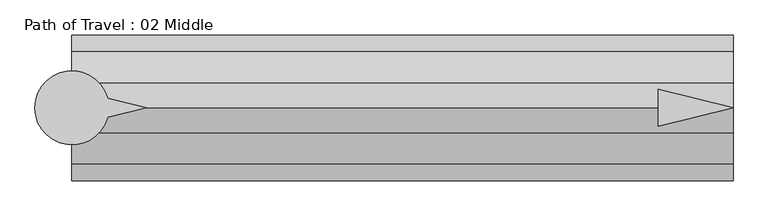
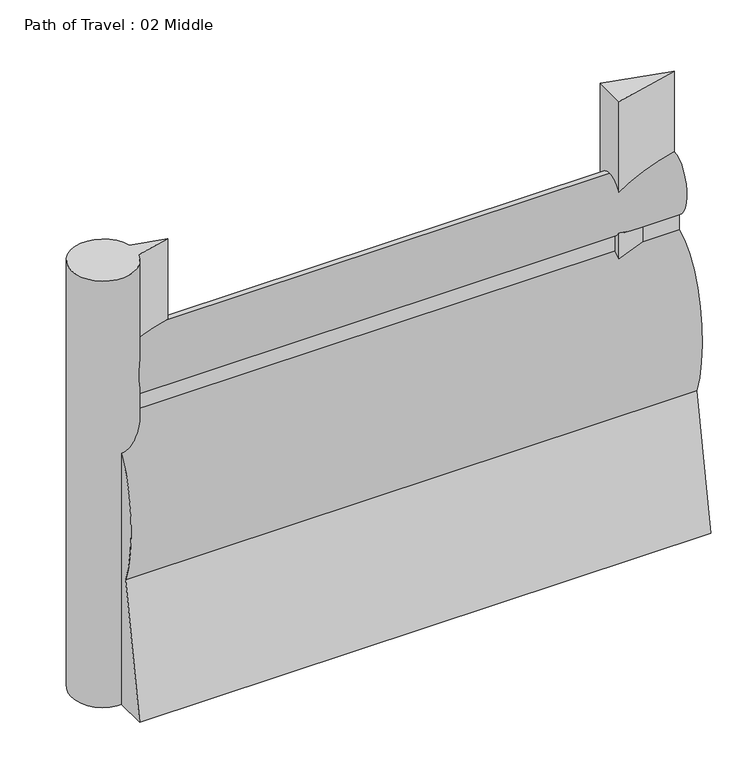
"""IFC4 building model written with IfcOpenShell, lengths in millimetres: proxy geometry, Path of Travel : 02 Middle."""

from ifc_helpers import new_model, si_unit, point, frame, frame_2d, origin, origin_with_axes, place, context, project, spatial, polyline, circle_curve, ellipse_curve, trimmed, segment, composite_curve, outline, extrude, source, transform, mapped, element, save
from ifc_brep_helpers import plane_surface, extruded_surface, advanced_brep


def path_of_travel_02_middle_6eefbcf4(model_context):
    return source(origin(), model_context, "Body", "SolidModel", [
        advanced_brep(
        [(227.5554837, 0.0, 1727.2), (227.5554837, 42.9018657, 1436.6534209), (227.5554837, 42.9018657, 1363.4763406), (227.5554837, 184.1186263, 643.4144547), (227.5554837, 297.5699544, 0.0), (227.5554837, 145.6574193, 0.0), (227.5554837, 0.0, 584.2), (227.5554837, -145.6574193, 0.0), (227.5554837, -297.5699544, 0.0), (227.5554837, -184.1186263, 643.4144547), (227.5554837, -42.9018657, 1363.4763406), (227.5554837, -42.9018657, 1436.6534209), (2925.8453525, 0.0, 1727.2), (2925.8453525, -42.9018657, 1436.6534209), (2925.8453525, -42.9018657, 1363.4763406), (2925.8453525, -184.1186263, 643.4144547), (2925.8453525, -297.5699544, 0.0), (2925.8453525, -145.6574193, 0.0), (2925.8453525, 0.0, 584.2), (2925.8453525, 145.6574193, 0.0), (2925.8453525, 297.5699544, 0.0), (2925.8453525, 184.1186263, 643.4144547), (2925.8453525, 42.9018657, 1363.4763406), (2925.8453525, 42.9018657, 1436.6534209)],
        [
            (0, 1, ellipse_curve(frame((227.5554837, 0.0, 1574.8), z_axis=(-1.0, 0.0, 0.0), x_axis=(0.0, 0.0, 1.0)), 152.4, 101.6)),
            (1, 2),
            (2, 3, ellipse_curve(frame((227.5554837, 0.0, 914.4), z_axis=(-1.0, 0.0, 0.0), x_axis=(0.0, 0.0, -1.0)), 457.2, 228.6)),
            (3, 4),
            (4, 5),
            (5, 6),
            (6, 7),
            (7, 8),
            (8, 9),
            (9, 10, ellipse_curve(frame((227.5554837, 0.0, 914.4), z_axis=(-1.0, 0.0, 0.0), x_axis=(0.0, 0.0, -1.0)), 457.2, 228.6)),
            (10, 11),
            (11, 0, ellipse_curve(frame((227.5554837, 0.0, 1574.8), z_axis=(-1.0, 0.0, 0.0), x_axis=(0.0, 0.0, 1.0)), 152.4, 101.6)),
            (12, 13, ellipse_curve(frame((2925.8453525, 0.0, 1574.8), z_axis=(1.0, 0.0, 0.0), x_axis=(0.0, 0.0, 1.0)), 152.4, 101.6)),
            (13, 14),
            (14, 15, ellipse_curve(frame((2925.8453525, 0.0, 914.4), z_axis=(1.0, 0.0, 0.0), x_axis=(0.0, 0.0, -1.0)), 457.2, 228.6)),
            (15, 16),
            (16, 17),
            (17, 18),
            (18, 19),
            (19, 20),
            (20, 21),
            (21, 22, ellipse_curve(frame((2925.8453525, 0.0, 914.4), z_axis=(1.0, 0.0, 0.0), x_axis=(0.0, 0.0, -1.0)), 457.2, 228.6)),
            (22, 23),
            (23, 12, ellipse_curve(frame((2925.8453525, 0.0, 1574.8), z_axis=(1.0, 0.0, 0.0), x_axis=(0.0, 0.0, 1.0)), 152.4, 101.6)),
            (0, 12),
            (23, 1),
            (22, 2),
            (21, 3),
            (20, 4),
            (19, 5),
            (18, 6),
            (17, 7),
            (16, 8),
            (15, 9),
            (14, 10),
            (13, 11),
        ],
        [
            plane_surface(frame((227.5554837, 0.0, 0.0), z_axis=(-1.0, 0.0, 0.0), x_axis=(0.0, 0.0, 1.0))),
            plane_surface(frame((2925.8453525, 0.0, 0.0), z_axis=(1.0, 0.0, 0.0), x_axis=(0.0, 0.0, 1.0))),
            extruded_surface(trimmed(ellipse_curve(frame((2925.8453525, 0.0, 1574.8), z_axis=(-1.0, 0.0, 0.0), x_axis=(0.0, 0.0, 1.0)), 152.4, 101.6), [point((2925.8453525, 0.0, 1727.2))], [point((2925.8453525, 42.9018657, 1436.6534209))], True, "CARTESIAN"), (-2698.2898688, 0.0, 0.0), 2698.2898688),
            plane_surface(frame((227.5554837, 42.9018657, 1436.6534209), z_axis=(0.0, 1.0, 0.0), x_axis=(1.0, 0.0, 0.0))),
            extruded_surface(trimmed(ellipse_curve(frame((2925.8453525, 0.0, 914.4), z_axis=(-1.0, 0.0, 0.0), x_axis=(0.0, 0.0, -1.0)), 457.2, 228.6), [point((2925.8453525, 42.9018657, 1363.4763406))], [point((2925.8453525, 184.1186263, 643.4144547))], True, "CARTESIAN"), (-2698.2898688, 0.0, 0.0), 2698.2898688),
            plane_surface(frame((227.5554837, 184.1186263, 643.4144547), z_axis=(0.0, 0.9848077530122078, 0.1736481776669322), x_axis=(1.0, 0.0, 0.0))),
            plane_surface(frame((227.5554837, 297.5699544, 0.0), z_axis=(0.0, 0.0, -1.0), x_axis=(1.0, 0.0, 0.0))),
            plane_surface(frame((227.5554837, 145.6574193, 0.0), z_axis=(0.0, -0.9702957262760199, -0.2419218955995739), x_axis=(1.0, 0.0, 0.0))),
            plane_surface(frame((227.5554837, 0.0, 584.2), z_axis=(0.0, 0.9702957262759961, -0.24192189559966923), x_axis=(1.0, 0.0, 0.0))),
            plane_surface(frame((227.5554837, -145.6574193, 0.0), z_axis=(0.0, 0.0, -1.0), x_axis=(1.0, 0.0, 0.0))),
            plane_surface(frame((227.5554837, -297.5699544, 0.0), z_axis=(0.0, -0.984807753012208, 0.17364817766693066), x_axis=(1.0, 0.0, 0.0))),
            extruded_surface(trimmed(ellipse_curve(frame((2925.8453525, 0.0, 914.4), z_axis=(-1.0, 0.0, 0.0), x_axis=(0.0, 0.0, -1.0)), 457.2, 228.6), [point((2925.8453525, -184.1186263, 643.4144547))], [point((2925.8453525, -42.9018657, 1363.4763406))], True, "CARTESIAN"), (-2698.2898688, 0.0, 0.0), 2698.2898688),
            plane_surface(frame((227.5554837, -42.9018657, 1363.4763406), z_axis=(0.0, -1.0, 0.0), x_axis=(1.0, 0.0, 0.0))),
            extruded_surface(trimmed(ellipse_curve(frame((2925.8453525, 0.0, 1574.8), z_axis=(-1.0, 0.0, 0.0), x_axis=(0.0, 0.0, 1.0)), 152.4, 101.6), [point((2925.8453525, -42.9018657, 1436.6534209))], [point((2925.8453525, 0.0, 1727.2))], True, "CARTESIAN"), (-2698.2898688, 0.0, 0.0), 2698.2898688),
        ],
        [
            (0, [[1, 2, 3, 4, 5, 6, 7, 8, 9, 10, 11, 12]]),
            (1, [[13, 14, 15, 16, 17, 18, 19, 20, 21, 22, 23, 24]]),
            (2, [[-1, 25, -24, 26]]),
            (3, [[-2, -26, -23, 27]]),
            (4, [[-3, -27, -22, 28]]),
            (5, [[-4, -28, -21, 29]]),
            (6, [[-5, -29, -20, 30]]),
            (7, [[-6, -30, -19, 31]]),
            (8, [[-7, -31, -18, 32]]),
            (9, [[-8, -32, -17, 33]]),
            (10, [[-9, -33, -16, 34]]),
            (11, [[-10, -34, -15, 35]]),
            (12, [[-11, -35, -14, 36]]),
            (13, [[-12, -36, -13, -25]]),
        ],
    ),
        extrude(outline(polyline([(2619.8402059, 76.2006338), (2925.8453525, 0.0), (2619.8402059, -76.2006338), (2619.8402059, 76.2006338)])), origin_with_axes(), (0.0, 0.0, 1.0), 2129.5973753),
        extrude(outline(composite_curve([segment(polyline([(372.7837828, 39.4440225), (531.182385, 0.0), (372.7837828, -39.4440225)]), True, "CONTINUOUS"), segment(trimmed(circle_curve(frame_2d((227.2200886, 0.0)), 150.8131956), [point((372.7837828, -39.4440225))], [point((372.7837828, 39.4440225))], False, "CARTESIAN"), True, "CONTINUOUS")], self_intersect=False)), origin_with_axes(), (0.0, 0.0, 1.0), 2129.5973753),
    ])


if __name__ == "__main__":
    model = new_model("IFC4")
    model_context = context("Model", 3, world=origin())
    ifc_project = project(units=[si_unit("LENGTHUNIT", "METRE", prefix="MILLI")], contexts=[model_context])
    site = spatial("IfcSite", under=ifc_project)
    building = spatial("IfcBuilding", under=site)
    placement = place(None, origin())
    path_of_travel_02_middle_shape = path_of_travel_02_middle_6eefbcf4(model_context)
    element("IfcBuildingElementProxy", 1, Name="Path of Travel : 02 Middle", ObjectType="Path of Travel : 02 Middle", at=placement, inside=building, context=model_context, shape_type="MappedRepresentation", body=[
        mapped(path_of_travel_02_middle_shape, transform((0.0, 0.0, 0.0), x_axis=(1.0, 0.0, 0.0), y_axis=(0.0, 1.0, 0.0), z_axis=(0.0, 0.0, 1.0))),
    ])
    save(model, "model.ifc")

# Revit data of these elements
# Type "Path of Travel : 02 Middle"
#   Path of Egress [instance default] = 4' - 0"
#   built-in parameter 1001306 [instance default] = 4 (stored number, unit not read)
#   Dot at Start = no
#   Arrow in Middle = yes
#   Arrow at End = no
#   Egress Path = none
# Element 1 (IfcBuildingElementProxy, "Path of Travel : 02 Middle")
#   Path of Egress = 8' - 10.23188"
#   built-in parameter 1001306 = 8.85266 (stored number, unit not read)
